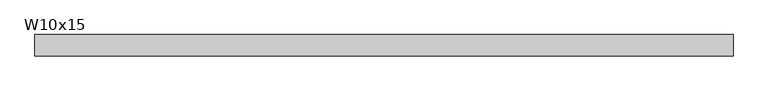
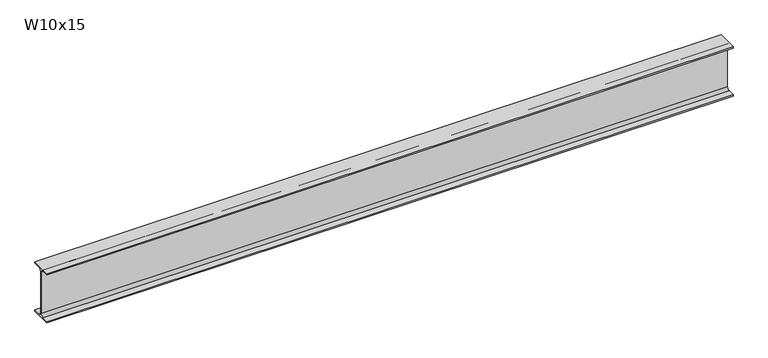
"""IFC4 building model written with IfcOpenShell, lengths in millimetres: beam geometry, RME W-Wide Flange : W10x15."""

import ifcopenshell
import ifcopenshell.guid

model = None  # the IFC model being written
_history = None  # IfcOwnerHistory: only IFC2X3 demands one
_inside = {}  # id of a spatial element -> (the spatial element, [elements in it])
_under = {}  # id of a project, library or spatial element -> (it, [spatial elements below it])
_declared = {}  # id of a project -> (the project, [libraries it declares])
_typed = {}  # id of a type object -> (the type object, [elements of that type])
_made_of = {}  # id of a material, layer set ... -> (it, [elements and type objects made of it])


def new_model(schema):
    """Start an empty IFC model of exactly this schema.

    Asked for "IFC4X3", IfcOpenShell would pick the latest addendum, in which some entities
    have other attributes; the version numbers below select the first issue.
    IFC2X3 requires an IfcOwnerHistory on every rooted entity: one is made here for all.
    """
    global model, _history
    if schema == "IFC4X3":
        model = ifcopenshell.file(schema_version=(4, 3, 0, 0))
    else:
        model = ifcopenshell.file(schema=schema)
    _inside.clear()
    _under.clear()
    _declared.clear()
    _typed.clear()
    _made_of.clear()
    _history = None
    if model.schema == "IFC2X3":
        org = make("IfcOrganization", Name="unknown")
        user = make(
            "IfcPersonAndOrganization",
            ThePerson=make("IfcPerson", FamilyName="unknown"),
            TheOrganization=org,
        )
        app = make(
            "IfcApplication",
            ApplicationDeveloper=org,
            Version="unknown",
            ApplicationFullName="unknown",
            ApplicationIdentifier="unknown",
        )
        _history = make(
            "IfcOwnerHistory",
            OwningUser=user,
            OwningApplication=app,
            ChangeAction="ADDED",
            CreationDate=0,
        )
    return model


def make(cls, **values):
    """One entity of the class cls with the attributes given. An attribute that is None is left unset."""
    return model.create_entity(
        cls, **{name: value for name, value in values.items() if value is not None}
    )


def rooted(cls, **values):
    """An entity with a GlobalId (a new one), such as an element, a storey or a relation."""
    return make(cls, GlobalId=ifcopenshell.guid.new(), OwnerHistory=_history, **values)


def si_unit(unit_type, name, prefix=None):
    """IfcSIUnit, for example si_unit("LENGTHUNIT", "METRE", prefix="MILLI")."""
    return make("IfcSIUnit", UnitType=unit_type, Prefix=prefix, Name=name)


def assignment(units):
    """IfcUnitAssignment: the units of a project."""
    return None if units is None else make("IfcUnitAssignment", Units=units)


def point(xyz):
    """IfcCartesianPoint."""
    return None if xyz is None else make("IfcCartesianPoint", Coordinates=xyz)


def direction(xyz):
    """IfcDirection."""
    return None if xyz is None else make("IfcDirection", DirectionRatios=xyz)


def frame(location, z_axis=None, x_axis=None):
    """IfcAxis2Placement3D, a coordinate frame: its origin and axes. An axis left out is left unset."""
    return make(
        "IfcAxis2Placement3D",
        Location=point(location),
        Axis=direction(z_axis),
        RefDirection=direction(x_axis),
    )


def frame_2d(location, x_axis=None):
    """IfcAxis2Placement2D, a coordinate frame in the plane: its origin and x axis."""
    return make(
        "IfcAxis2Placement2D", Location=point(location), RefDirection=direction(x_axis)
    )


def origin():
    """The frame at (0, 0, 0) with its axes left unset."""
    return frame((0.0, 0.0, 0.0))


def place(relative_to, where):
    """IfcLocalPlacement: puts the frame where relative to a parent placement (None: the world)."""
    return make(
        "IfcLocalPlacement", PlacementRelTo=relative_to, RelativePlacement=where
    )


def context(
    kind, dimensions, precision=None, world=None, true_north=None, identifier=None
):
    """IfcGeometricRepresentationContext, for example the 3D "Model" context."""
    return make(
        "IfcGeometricRepresentationContext",
        ContextIdentifier=identifier,
        ContextType=kind,
        CoordinateSpaceDimension=dimensions,
        Precision=precision,
        WorldCoordinateSystem=world,
        TrueNorth=true_north,
    )


def project(units=None, contexts=None):
    """IfcProject with its units and contexts."""
    return rooted(
        "IfcProject",
        Name="project",
        RepresentationContexts=contexts,
        UnitsInContext=assignment(units),
    )


def spatial(cls, under=None, at=None, **own):
    """A site, building, storey or space (cls), placed at a placement, below another one or the project."""
    s = rooted(cls, ObjectPlacement=at, **own)
    if under is not None:
        _under.setdefault(under.id(), (under, []))[1].append(s)
    return s


def polyline(points):
    """IfcPolyline through the points."""
    return make("IfcPolyline", Points=[point(p) for p in points])


def circle_curve(where, radius):
    """IfcCircle in the frame where."""
    return make("IfcCircle", Position=where, Radius=radius)


def trimmed(basis, trim1, trim2, sense, master):
    """IfcTrimmedCurve: the piece of a basis curve between two trims."""
    return make(
        "IfcTrimmedCurve",
        BasisCurve=basis,
        Trim1=trim1,
        Trim2=trim2,
        SenseAgreement=sense,
        MasterRepresentation=master,
    )


def segment(curve, same_sense, transition):
    """IfcCompositeCurveSegment."""
    return make(
        "IfcCompositeCurveSegment",
        Transition=transition,
        SameSense=same_sense,
        ParentCurve=curve,
    )


def composite_curve(segments, self_intersect=None):
    """IfcCompositeCurve: segments joined end to end."""
    return make("IfcCompositeCurve", Segments=segments, SelfIntersect=self_intersect)


def outline(outer, holes=None, kind="AREA"):
    """IfcArbitraryClosedProfileDef: a profile drawn as a closed curve; with holes, ...WithVoids."""
    if holes is None:
        return make("IfcArbitraryClosedProfileDef", ProfileType=kind, OuterCurve=outer)
    return make(
        "IfcArbitraryProfileDefWithVoids",
        ProfileType=kind,
        OuterCurve=outer,
        InnerCurves=holes,
    )


def extrude(swept, where, along, depth):
    """IfcExtrudedAreaSolid: the profile swept, set in the frame where, extruded along a direction by depth."""
    return make(
        "IfcExtrudedAreaSolid",
        SweptArea=swept,
        Position=where,
        ExtrudedDirection=direction(along),
        Depth=depth,
    )


def shape(context_of_items, identifier, shape_type, items):
    """IfcShapeRepresentation: the items that make up one representation, for example the "Body"."""
    return make(
        "IfcShapeRepresentation",
        ContextOfItems=context_of_items,
        RepresentationIdentifier=identifier,
        RepresentationType=shape_type,
        Items=items,
    )


def source(mapping_origin, context_of_items, identifier, shape_type, items):
    """IfcRepresentationMap: a shape defined once, which mapped items show again and again."""
    return make(
        "IfcRepresentationMap",
        MappingOrigin=mapping_origin,
        MappedRepresentation=shape(context_of_items, identifier, shape_type, items),
    )


def transform(
    local_origin,
    x_axis=None,
    y_axis=None,
    z_axis=None,
    scale=None,
    scale2=None,
    scale3=None,
    uniform=True,
):
    """IfcCartesianTransformationOperator3D, or its non-uniform kind. x_axis, y_axis, z_axis: its Axis1, 2, 3."""
    if uniform:
        return make(
            "IfcCartesianTransformationOperator3D",
            Axis1=direction(x_axis),
            Axis2=direction(y_axis),
            LocalOrigin=point(local_origin),
            Scale=scale,
            Axis3=direction(z_axis),
        )
    return make(
        "IfcCartesianTransformationOperator3DnonUniform",
        Axis1=direction(x_axis),
        Axis2=direction(y_axis),
        LocalOrigin=point(local_origin),
        Scale=scale,
        Axis3=direction(z_axis),
        Scale2=scale2,
        Scale3=scale3,
    )


def mapped(mapping_source, mapping_target):
    """IfcMappedItem: shows the shape of a source again, moved by a transform."""
    return make(
        "IfcMappedItem", MappingSource=mapping_source, MappingTarget=mapping_target
    )


def made_of(thing, what):
    """Note that an element or type object is made of a material, layer set ...; save() writes the relation."""
    if what is not None:
        _made_of.setdefault(what.id(), (what, []))[1].append(thing)
    return thing


def element(
    cls,
    number,
    at=None,
    inside=None,
    cuts=None,
    type_object=None,
    material=None,
    context=None,
    identifier="Body",
    shape_type=None,
    held_by="IfcProductDefinitionShape",
    body=None,
    shapes=None,
    **own,
):
    """One element of the class cls, such as IfcWall. Its Tag is "e" and its number.

    at: its placement. inside: the storey or other place that contains it. cuts: it is an
    opening in that element (IfcRelVoidsElement). A single representation is given by context,
    identifier, shape_type and body (its items); several are given by shapes. held_by: the class
    of the entity that holds the representations. save() writes the other relations.
    """
    e = rooted(cls, Tag="e%d" % number, ObjectPlacement=at, **own)
    if body is not None:
        shapes = [shape(context, identifier, shape_type, body)]
    if shapes is not None:
        e.Representation = make(held_by, Representations=shapes)
    if inside is not None:
        _inside.setdefault(inside.id(), (inside, []))[1].append(e)
    if cuts is not None:
        rooted(
            "IfcRelVoidsElement", RelatingBuildingElement=cuts, RelatedOpeningElement=e
        )
    if type_object is not None:
        _typed.setdefault(type_object.id(), (type_object, []))[1].append(e)
    return made_of(e, material)


def aggregate(whole, parts):
    """IfcRelAggregates: a whole, such as a stair, and the parts it consists of."""
    return rooted("IfcRelAggregates", RelatingObject=whole, RelatedObjects=parts)


def save(model, path):
    """Write the relations noted so far, then the file.

    IfcRelAggregates (storeys below a building ...), IfcRelContainedInSpatialStructure (elements
    in a storey), IfcRelDefinesByType, IfcRelAssociatesMaterial and IfcRelDeclares: one each for
    every whole, place, type object, material and project.
    """
    for whole, parts in _under.values():
        aggregate(whole, parts)
    for where, things in _inside.values():
        rooted(
            "IfcRelContainedInSpatialStructure",
            RelatedElements=things,
            RelatingStructure=where,
        )
    for kind, things in _typed.values():
        rooted("IfcRelDefinesByType", RelatedObjects=things, RelatingType=kind)
    for what, things in _made_of.values():
        rooted("IfcRelAssociatesMaterial", RelatedObjects=things, RelatingMaterial=what)
    for by, libraries in _declared.values():
        rooted("IfcRelDeclares", RelatingContext=by, RelatedDefinitions=libraries)
    model.write(path)


def w10x15_5ca210f8(model_context):
    return source(origin(), model_context, "Body", "SweptSolid", [
        extrude(outline(composite_curve([segment(polyline([(50.8, -120.142), (50.8, -127.0), (-50.8, -127.0), (-50.8, -120.142), (-16.7005, -120.142)]), True, "CONTINUOUS"), segment(trimmed(circle_curve(frame_2d((-16.7005, -106.3625)), 13.7795), [point((-16.7005, -120.142))], [point((-2.921, -106.3625))], True, "CARTESIAN"), True, "CONTINUOUS"), segment(polyline([(-2.921, -106.3625), (-2.921, 106.3625)]), True, "CONTINUOUS"), segment(trimmed(circle_curve(frame_2d((-16.7005, 106.3625)), 13.7795), [point((-2.921, 106.3625))], [point((-16.7005, 120.142))], True, "CARTESIAN"), True, "CONTINUOUS"), segment(polyline([(-16.7005, 120.142), (-50.8, 120.142), (-50.8, 127.0), (50.8, 127.0), (50.8, 120.142), (16.7005, 120.142)]), True, "CONTINUOUS"), segment(trimmed(circle_curve(frame_2d((16.7005, 106.3625)), 13.7795), [point((16.7005, 120.142))], [point((2.921, 106.3625))], True, "CARTESIAN"), True, "CONTINUOUS"), segment(polyline([(2.921, 106.3625), (2.921, -106.3625)]), True, "CONTINUOUS"), segment(trimmed(circle_curve(frame_2d((16.7005, -106.3625)), 13.7795), [point((2.921, -106.3625))], [point((16.7005, -120.142))], True, "CARTESIAN"), True, "CONTINUOUS"), segment(polyline([(16.7005, -120.142), (50.8, -120.142)]), True, "CONTINUOUS")], self_intersect=False)), frame((-1668.6182178, 0.0, 0.0), z_axis=(1.0, 0.0, 0.0), x_axis=(0.0, 1.0, 0.0)), (0.0, 0.0, 1.0), 3337.2364356),
    ])


if __name__ == "__main__":
    model = new_model("IFC4")
    model_context = context("Model", 3, world=origin())
    ifc_project = project(units=[si_unit("LENGTHUNIT", "METRE", prefix="MILLI")], contexts=[model_context])
    site = spatial("IfcSite", under=ifc_project)
    building = spatial("IfcBuilding", under=site)
    placement = place(None, origin())
    w10x15_shape = w10x15_5ca210f8(model_context)
    element("IfcBeam", 1, ObjectType="RME W-Wide Flange : W10x15", at=placement, inside=building, context=model_context, shape_type="MappedRepresentation", body=[
        mapped(w10x15_shape, transform((0.0, 0.0, 0.0), x_axis=(1.0, 0.0, 0.0), y_axis=(0.0, 1.0, 0.0), z_axis=(0.0, 0.0, 1.0))),
    ])
    save(model, "model.ifc")

# Revit data of these elements
# Type "RME W-Wide Flange : W10x15"
#   WELD P [instance default] = ""
#   WELD LE [instance default] = ""
#   WELD D [instance default] = ""
#   TOP SECTION SIZE [instance default] = ""
#   TOP SECTION LENGTH [instance default] = ""
#   REMARKS [instance default] = ""
#   REINF TYPE [instance default] = ""
#   Nominal Size = "W24"
#   End Bearing Capacity [instance default] = ""
#   BOT SECTION SIZE [instance default] = ""
#   BOT SECTION LENGTH [instance default] = ""
#   Assembly Code = "B10"
#   W = 15
#   Start Extension Calculation [instance default] = 10' - 0"
#   Start Extension [instance default] = -0' - 0 1/2"
#   End Extension Calculation [instance default] = 10' - 0"
#   End Extension [instance default] = -0' - 0 1/2"
#   Length [instance default] = 5' - 0"
#   bf = 0' - 4"
#   d = 0' - 10"
#   k = 0' - 0 13/16"
#   k2 = 0' - 0.5425"
#   tf = 0' - 0.27"
#   tw = 0' - 0.23"
#   A = 0.030625 SF
#   Structural Material [instance default] = Metal - Steel - ASTM A992
# Element 1 (IfcBeam, "RME W-Wide Flange : W10x15")
#   Length = 10' - 11.38726"
#   Materials on its faces: "Metal - Steel - ASTM A992"
# Materials
#   "Metal - Steel - ASTM A992": class "Metal", colour RGB 255 128 0, transparency 0
